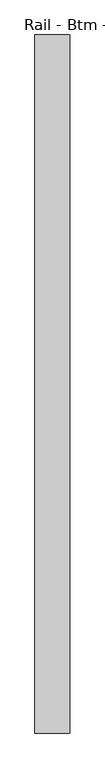
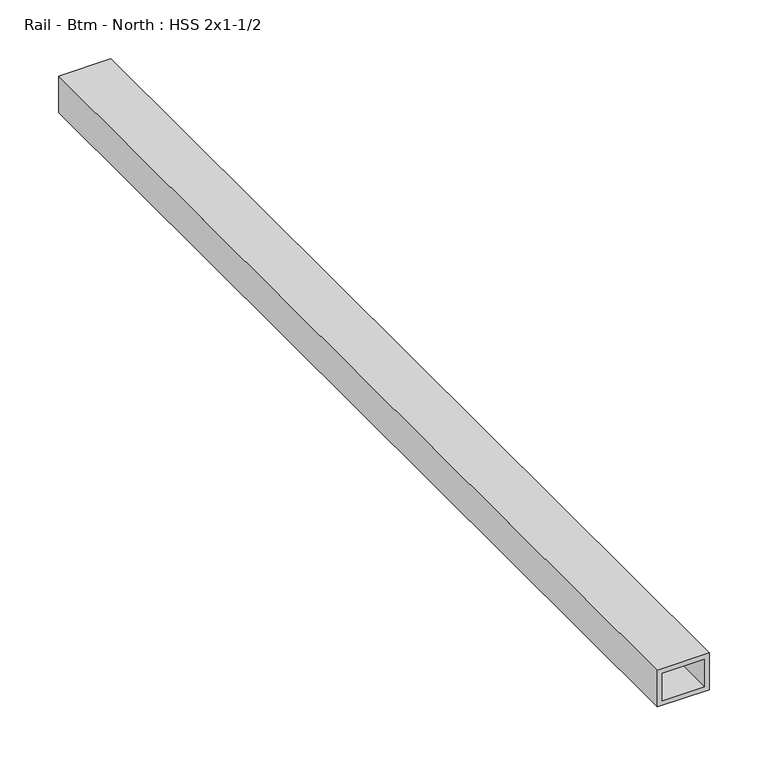
"""IFC4 building model written with IfcOpenShell, lengths in millimetres: proxy geometry, Rail - Btm - North : HSS 2x1-1/2."""

from ifc_helpers import new_model, si_unit, frame, origin, place, context, project, spatial, polyline, outline, extrude, source, transform, mapped, element, save


def rail_btm_north_hss_2x1_1_2_b7e517c1(model_context):
    return source(origin(), model_context, "Body", "SweptSolid", [
        extrude(outline(polyline([(50.8, 587416.6934739), (88.9, 587416.6934739), (88.9, 587365.8934739), (50.8, 587365.8934739), (50.8, 587416.6934739)]), holes=[polyline([(84.1375, 587411.9309739), (55.5625, 587411.9309739), (55.5625, 587370.6559739), (84.1375, 587370.6559739), (84.1375, 587411.9309739)])]), frame((0.0, -532839.3663841, 0.0), z_axis=(0.0, 1.0, 0.0), x_axis=(0.0, 0.0, 1.0)), (0.0, 0.0, 1.0), 1016.0),
    ])


if __name__ == "__main__":
    model = new_model("IFC4")
    model_context = context("Model", 3, world=origin())
    ifc_project = project(units=[si_unit("LENGTHUNIT", "METRE", prefix="MILLI")], contexts=[model_context])
    site = spatial("IfcSite", under=ifc_project)
    building = spatial("IfcBuilding", under=site)
    placement = place(None, origin())
    rail_btm_north_hss_2x1_1_2_shape = rail_btm_north_hss_2x1_1_2_b7e517c1(model_context)
    element("IfcBuildingElementProxy", 1, Name="Rail - Btm - North : HSS 2x1-1/2", ObjectType="Rail - Btm - North : HSS 2x1-1/2", at=placement, inside=building, context=model_context, shape_type="MappedRepresentation", body=[
        mapped(rail_btm_north_hss_2x1_1_2_shape, transform((0.0, 0.0, 0.0), x_axis=(1.0, 0.0, 0.0), y_axis=(0.0, 1.0, 0.0), z_axis=(0.0, 0.0, 1.0))),
    ])
    save(model, "model.ifc")

# Revit data of these elements
# Element 1 (IfcBuildingElementProxy, "Rail - Btm - North : HSS 2x1-1/2")
#   Materials on its faces: "1-1/2\"X2\" GALV. STL HSS TUBING"
# Materials
#   "1-1/2\"X2\" GALV. STL HSS TUBING": class "Generic", colour RGB 211 211 207, transparency 0, Cost = 0
